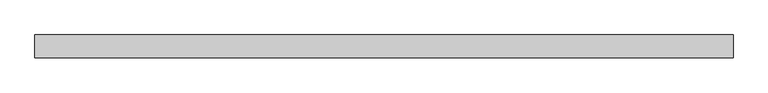
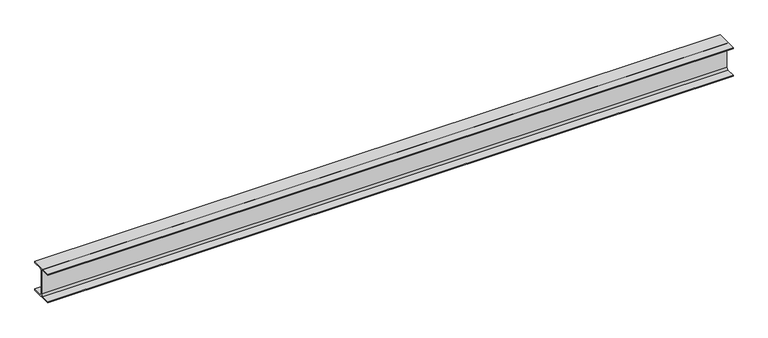
"""IFC4 building model written with IfcOpenShell, lengths in millimetres: beam geometry, 0912_Steel Framing_H-KSD3502 : H_SB_ASB_H-340x250x9x14."""

from ifc_helpers import new_model, si_unit, point, frame, frame_2d, origin, place, context, project, spatial, polyline, circle_curve, trimmed, segment, composite_curve, outline, extrude, source, transform, mapped, element, save


def beam_f14934d3(model_context):
    return source(origin(), model_context, "Body", "SweptSolid", [
        extrude(outline(composite_curve([segment(polyline([(125.0, -156.0), (125.0, -170.0), (-125.0, -170.0), (-125.0, -156.0), (-24.5, -156.0)]), True, "CONTINUOUS"), segment(trimmed(circle_curve(frame_2d((-24.5, -136.0)), 20.0), [point((-24.5, -156.0))], [point((-4.5, -136.0))], True, "CARTESIAN"), True, "CONTINUOUS"), segment(polyline([(-4.5, -136.0), (-4.5, 136.0)]), True, "CONTINUOUS"), segment(trimmed(circle_curve(frame_2d((-24.5, 136.0)), 20.0), [point((-4.5, 136.0))], [point((-24.5, 156.0))], True, "CARTESIAN"), True, "CONTINUOUS"), segment(polyline([(-24.5, 156.0), (-125.0, 156.0), (-125.0, 170.0), (125.0, 170.0), (125.0, 156.0), (24.5, 156.0)]), True, "CONTINUOUS"), segment(trimmed(circle_curve(frame_2d((24.5, 136.0)), 20.0), [point((24.5, 156.0))], [point((4.5, 136.0))], True, "CARTESIAN"), True, "CONTINUOUS"), segment(polyline([(4.5, 136.0), (4.5, -136.0)]), True, "CONTINUOUS"), segment(trimmed(circle_curve(frame_2d((24.5, -136.0)), 20.0), [point((4.5, -136.0))], [point((24.5, -156.0))], True, "CARTESIAN"), True, "CONTINUOUS"), segment(polyline([(24.5, -156.0), (125.0, -156.0)]), True, "CONTINUOUS")], self_intersect=False)), frame((-3837.3, 0.0, 0.0), z_axis=(1.0, 0.0, 0.0), x_axis=(0.0, 1.0, 0.0)), (0.0, 0.0, 1.0), 7674.6),
    ])


if __name__ == "__main__":
    model = new_model("IFC4")
    model_context = context("Model", 3, world=origin())
    ifc_project = project(units=[si_unit("LENGTHUNIT", "METRE", prefix="MILLI")], contexts=[model_context])
    site = spatial("IfcSite", under=ifc_project)
    building = spatial("IfcBuilding", under=site)
    placement = place(None, origin())
    beam_shape = beam_f14934d3(model_context)
    element("IfcBeam", 1, ObjectType="0912_Steel Framing_H-KSD3502 : H_SB_ASB_H-340x250x9x14", at=placement, inside=building, context=model_context, shape_type="MappedRepresentation", body=[
        mapped(beam_shape, transform((0.0, 0.0, 0.0), x_axis=(1.0, 0.0, 0.0), y_axis=(0.0, 1.0, 0.0), z_axis=(0.0, 0.0, 1.0))),
    ])
    save(model, "model.ifc")

# Revit data of these elements
# Type "0912_Steel Framing_H-KSD3502 : H_SB_ASB_H-340x250x9x14"
#   H_WM Code_1 = "S01AA002-00001 | Main Steel Structure Fabrication Work | Shelter/Building | Medium Steel - Standard (90KG/M>Weight≥30KG/M) | Material: (   )"
#   H_WM Code_2 = "S03AA028-00001 | Main Steel Structure Erection Work | Shelter/Building | Medium Steel (90KG/M>Weight≥30KG/M) | Material: (   )"
#   H_WM Code_3 = "S01AA010-00001 | Main Steel Structure Fabrication Work | Shelter/Building | Steel Painting/Coating | for Non-Fireproofed Steel Surface, Surface Preparation, Primer, Second & Final Coat | Material: (   )"
#   H_Q'ty Cal Type Tag = "SB-Q2"
#   Width = 25.0 cm
#   Web Thickness = 0.9 cm
#   Web Fillet = 2.0 cm
#   Warping Constant = 969000.0 cm⁶
#   W = 0
#   Torsional Moment of Inertia = 53.6551 cm⁴
#   Section Area = 101.5 cm²
#   Plastic Modulus weak axis = 447.0 cm³
#   Plastic Modulus strong axis = 1410.0 cm³
#   Perimeter = 1.63 m²/m
#   Nominal Weight = 79.70 kgf/m
#   Moment of Inertia weak axis = 3650.00 cm⁴
#   Moment of Inertia strong axis = 21700.00 cm⁴
#   Height = 34.0 cm
#   Flange Thickness = 1.4 cm
#   Elastic Modulus weak axis = 292.0 cm³
#   Elastic Modulus strong axis = 1280.0 cm³
#   Centroid Vertical = 17.0 cm
#   Centroid Horizontal = 12.5 cm
#   Ix = 217000000
#   Length [instance default] = 1.5240 m
#   Zx = 1410000
#   b = 0.2500 m
#   h = 0.3400 m
#   r = 0.0200 m
#   s = 0.0090 m
#   t = 0.0140 m
#   A = 0.01015 m²
#   Structural Material [instance default] = Steel, 45-345
#   Assembly Code = ""
# Element 1 (IfcBeam, "0912_Steel Framing_H-KSD3502 : H_SB_ASB_H-340x250x9x14")
#   Structural Material = none
# Materials
#   "Steel, 45-345": class "Metal", colour RGB 189 187 185, transparency 0, Description = "Steel 345 MPa", Cost = 0
